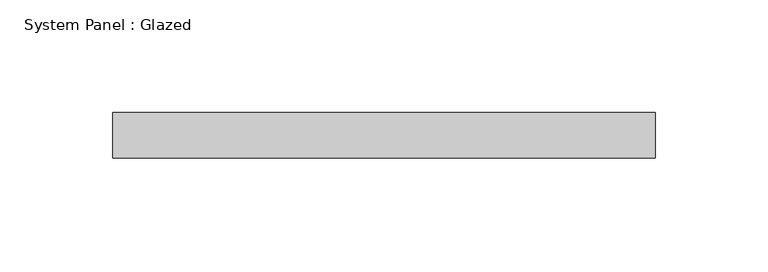
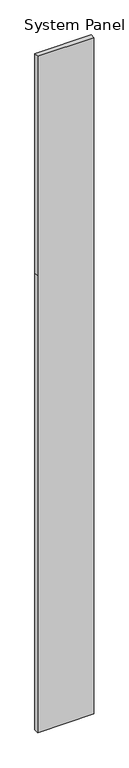
"""IFC4 building model written with IfcOpenShell, lengths in millimetres: plate geometry, System Panel : Glazed."""

import ifcopenshell
import ifcopenshell.guid

model = None  # the IFC model being written
_history = None  # IfcOwnerHistory: only IFC2X3 demands one
_inside = {}  # id of a spatial element -> (the spatial element, [elements in it])
_under = {}  # id of a project, library or spatial element -> (it, [spatial elements below it])
_declared = {}  # id of a project -> (the project, [libraries it declares])
_typed = {}  # id of a type object -> (the type object, [elements of that type])
_made_of = {}  # id of a material, layer set ... -> (it, [elements and type objects made of it])


def new_model(schema):
    """Start an empty IFC model of exactly this schema.

    Asked for "IFC4X3", IfcOpenShell would pick the latest addendum, in which some entities
    have other attributes; the version numbers below select the first issue.
    IFC2X3 requires an IfcOwnerHistory on every rooted entity: one is made here for all.
    """
    global model, _history
    if schema == "IFC4X3":
        model = ifcopenshell.file(schema_version=(4, 3, 0, 0))
    else:
        model = ifcopenshell.file(schema=schema)
    _inside.clear()
    _under.clear()
    _declared.clear()
    _typed.clear()
    _made_of.clear()
    _history = None
    if model.schema == "IFC2X3":
        org = make("IfcOrganization", Name="unknown")
        user = make(
            "IfcPersonAndOrganization",
            ThePerson=make("IfcPerson", FamilyName="unknown"),
            TheOrganization=org,
        )
        app = make(
            "IfcApplication",
            ApplicationDeveloper=org,
            Version="unknown",
            ApplicationFullName="unknown",
            ApplicationIdentifier="unknown",
        )
        _history = make(
            "IfcOwnerHistory",
            OwningUser=user,
            OwningApplication=app,
            ChangeAction="ADDED",
            CreationDate=0,
        )
    return model


def make(cls, **values):
    """One entity of the class cls with the attributes given. An attribute that is None is left unset."""
    return model.create_entity(
        cls, **{name: value for name, value in values.items() if value is not None}
    )


def rooted(cls, **values):
    """An entity with a GlobalId (a new one), such as an element, a storey or a relation."""
    return make(cls, GlobalId=ifcopenshell.guid.new(), OwnerHistory=_history, **values)


def si_unit(unit_type, name, prefix=None):
    """IfcSIUnit, for example si_unit("LENGTHUNIT", "METRE", prefix="MILLI")."""
    return make("IfcSIUnit", UnitType=unit_type, Prefix=prefix, Name=name)


def assignment(units):
    """IfcUnitAssignment: the units of a project."""
    return None if units is None else make("IfcUnitAssignment", Units=units)


def point(xyz):
    """IfcCartesianPoint."""
    return None if xyz is None else make("IfcCartesianPoint", Coordinates=xyz)


def direction(xyz):
    """IfcDirection."""
    return None if xyz is None else make("IfcDirection", DirectionRatios=xyz)


def frame(location, z_axis=None, x_axis=None):
    """IfcAxis2Placement3D, a coordinate frame: its origin and axes. An axis left out is left unset."""
    return make(
        "IfcAxis2Placement3D",
        Location=point(location),
        Axis=direction(z_axis),
        RefDirection=direction(x_axis),
    )


def origin():
    """The frame at (0, 0, 0) with its axes left unset."""
    return frame((0.0, 0.0, 0.0))


def place(relative_to, where):
    """IfcLocalPlacement: puts the frame where relative to a parent placement (None: the world)."""
    return make(
        "IfcLocalPlacement", PlacementRelTo=relative_to, RelativePlacement=where
    )


def context(
    kind, dimensions, precision=None, world=None, true_north=None, identifier=None
):
    """IfcGeometricRepresentationContext, for example the 3D "Model" context."""
    return make(
        "IfcGeometricRepresentationContext",
        ContextIdentifier=identifier,
        ContextType=kind,
        CoordinateSpaceDimension=dimensions,
        Precision=precision,
        WorldCoordinateSystem=world,
        TrueNorth=true_north,
    )


def project(units=None, contexts=None):
    """IfcProject with its units and contexts."""
    return rooted(
        "IfcProject",
        Name="project",
        RepresentationContexts=contexts,
        UnitsInContext=assignment(units),
    )


def spatial(cls, under=None, at=None, **own):
    """A site, building, storey or space (cls), placed at a placement, below another one or the project."""
    s = rooted(cls, ObjectPlacement=at, **own)
    if under is not None:
        _under.setdefault(under.id(), (under, []))[1].append(s)
    return s


def polyline(points):
    """IfcPolyline through the points."""
    return make("IfcPolyline", Points=[point(p) for p in points])


def outline(outer, holes=None, kind="AREA"):
    """IfcArbitraryClosedProfileDef: a profile drawn as a closed curve; with holes, ...WithVoids."""
    if holes is None:
        return make("IfcArbitraryClosedProfileDef", ProfileType=kind, OuterCurve=outer)
    return make(
        "IfcArbitraryProfileDefWithVoids",
        ProfileType=kind,
        OuterCurve=outer,
        InnerCurves=holes,
    )


def extrude(swept, where, along, depth):
    """IfcExtrudedAreaSolid: the profile swept, set in the frame where, extruded along a direction by depth."""
    return make(
        "IfcExtrudedAreaSolid",
        SweptArea=swept,
        Position=where,
        ExtrudedDirection=direction(along),
        Depth=depth,
    )


def shape(context_of_items, identifier, shape_type, items):
    """IfcShapeRepresentation: the items that make up one representation, for example the "Body"."""
    return make(
        "IfcShapeRepresentation",
        ContextOfItems=context_of_items,
        RepresentationIdentifier=identifier,
        RepresentationType=shape_type,
        Items=items,
    )


def source(mapping_origin, context_of_items, identifier, shape_type, items):
    """IfcRepresentationMap: a shape defined once, which mapped items show again and again."""
    return make(
        "IfcRepresentationMap",
        MappingOrigin=mapping_origin,
        MappedRepresentation=shape(context_of_items, identifier, shape_type, items),
    )


def transform(
    local_origin,
    x_axis=None,
    y_axis=None,
    z_axis=None,
    scale=None,
    scale2=None,
    scale3=None,
    uniform=True,
):
    """IfcCartesianTransformationOperator3D, or its non-uniform kind. x_axis, y_axis, z_axis: its Axis1, 2, 3."""
    if uniform:
        return make(
            "IfcCartesianTransformationOperator3D",
            Axis1=direction(x_axis),
            Axis2=direction(y_axis),
            LocalOrigin=point(local_origin),
            Scale=scale,
            Axis3=direction(z_axis),
        )
    return make(
        "IfcCartesianTransformationOperator3DnonUniform",
        Axis1=direction(x_axis),
        Axis2=direction(y_axis),
        LocalOrigin=point(local_origin),
        Scale=scale,
        Axis3=direction(z_axis),
        Scale2=scale2,
        Scale3=scale3,
    )


def mapped(mapping_source, mapping_target):
    """IfcMappedItem: shows the shape of a source again, moved by a transform."""
    return make(
        "IfcMappedItem", MappingSource=mapping_source, MappingTarget=mapping_target
    )


def made_of(thing, what):
    """Note that an element or type object is made of a material, layer set ...; save() writes the relation."""
    if what is not None:
        _made_of.setdefault(what.id(), (what, []))[1].append(thing)
    return thing


def element(
    cls,
    number,
    at=None,
    inside=None,
    cuts=None,
    type_object=None,
    material=None,
    context=None,
    identifier="Body",
    shape_type=None,
    held_by="IfcProductDefinitionShape",
    body=None,
    shapes=None,
    **own,
):
    """One element of the class cls, such as IfcWall. Its Tag is "e" and its number.

    at: its placement. inside: the storey or other place that contains it. cuts: it is an
    opening in that element (IfcRelVoidsElement). A single representation is given by context,
    identifier, shape_type and body (its items); several are given by shapes. held_by: the class
    of the entity that holds the representations. save() writes the other relations.
    """
    e = rooted(cls, Tag="e%d" % number, ObjectPlacement=at, **own)
    if body is not None:
        shapes = [shape(context, identifier, shape_type, body)]
    if shapes is not None:
        e.Representation = make(held_by, Representations=shapes)
    if inside is not None:
        _inside.setdefault(inside.id(), (inside, []))[1].append(e)
    if cuts is not None:
        rooted(
            "IfcRelVoidsElement", RelatingBuildingElement=cuts, RelatedOpeningElement=e
        )
    if type_object is not None:
        _typed.setdefault(type_object.id(), (type_object, []))[1].append(e)
    return made_of(e, material)


def aggregate(whole, parts):
    """IfcRelAggregates: a whole, such as a stair, and the parts it consists of."""
    return rooted("IfcRelAggregates", RelatingObject=whole, RelatedObjects=parts)


def save(model, path):
    """Write the relations noted so far, then the file.

    IfcRelAggregates (storeys below a building ...), IfcRelContainedInSpatialStructure (elements
    in a storey), IfcRelDefinesByType, IfcRelAssociatesMaterial and IfcRelDeclares: one each for
    every whole, place, type object, material and project.
    """
    for whole, parts in _under.values():
        aggregate(whole, parts)
    for where, things in _inside.values():
        rooted(
            "IfcRelContainedInSpatialStructure",
            RelatedElements=things,
            RelatingStructure=where,
        )
    for kind, things in _typed.values():
        rooted("IfcRelDefinesByType", RelatedObjects=things, RelatingType=kind)
    for what, things in _made_of.values():
        rooted("IfcRelAssociatesMaterial", RelatedObjects=things, RelatingMaterial=what)
    for by, libraries in _declared.values():
        rooted("IfcRelDeclares", RelatingContext=by, RelatedDefinitions=libraries)
    model.write(path)


def system_panel_glazed_c7de043b(model_context):
    return source(origin(), model_context, "Body", "SweptSolid", [
        extrude(outline(polyline([(0.0, -120.0), (0.0, 120.0), (2060.0, 120.0), (3050.0, 120.0), (3050.0, -120.0), (2060.0, -120.0), (0.0, -120.0)])), frame((0.0, 0.0, 0.0), z_axis=(0.0, 1.0, 0.0), x_axis=(0.0, 0.0, 1.0)), (0.0, 0.0, 1.0), 20.0),
    ])


if __name__ == "__main__":
    model = new_model("IFC4")
    model_context = context("Model", 3, world=origin())
    ifc_project = project(units=[si_unit("LENGTHUNIT", "METRE", prefix="MILLI")], contexts=[model_context])
    site = spatial("IfcSite", under=ifc_project)
    building = spatial("IfcBuilding", under=site)
    placement = place(None, origin())
    system_panel_glazed_shape = system_panel_glazed_c7de043b(model_context)
    element("IfcPlate", 1, ObjectType="System Panel : Glazed", at=placement, inside=building, context=model_context, shape_type="MappedRepresentation", body=[
        mapped(system_panel_glazed_shape, transform((0.0, 0.0, 0.0), x_axis=(1.0, 0.0, 0.0), y_axis=(0.0, 1.0, 0.0), z_axis=(0.0, 0.0, 1.0))),
    ])
    save(model, "model.ifc")

# Revit data of these elements
# Type "System Panel : Glazed"
#   COBie.Type = no
# Element 1 (IfcPlate, "System Panel : Glazed")
#   Materials on its faces: "Glass"
# Materials
#   "Glass": class "Glass", colour RGB 0 128 192, transparency 0.75, Description = "Soda Lime Glass", Cost = 0
